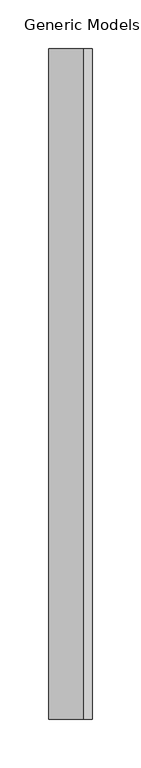
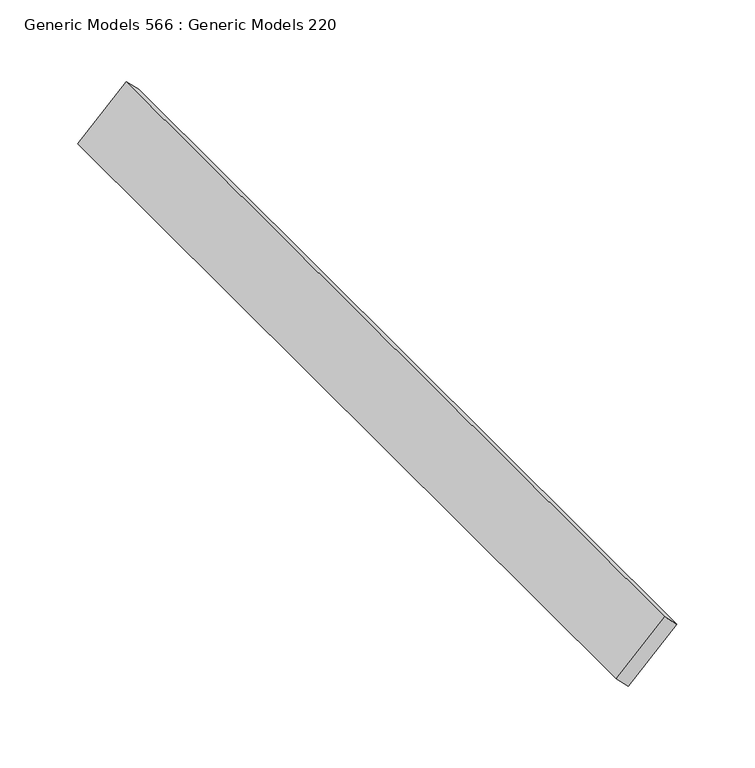
"""IFC4 building model written with IfcOpenShell, lengths in millimetres: proxy geometry, Generic Models 566 : Generic Models 220."""

from ifc_helpers import new_model, si_unit, frame, origin, place, context, project, spatial, polyline, outline, extrude, source, transform, mapped, element, save


def generic_models_566_generic_models_220_5707b333(model_context):
    return source(origin(), model_context, "Body", "SweptSolid", [
        extrude(outline(polyline([(0.0, -12.7000001), (0.0, 0.0), (690.8142348, 0.0), (690.8142348, -12.7000001), (0.0, -12.7000001)])), frame((7841.3059863, 4539.4872686, 124176.1399101), z_axis=(0.7071067811868034, 0.0, 0.7071067811862918), x_axis=(0.0, -1.0, 0.0)), (0.0, 0.0, 1.0), 50.8),
    ])


if __name__ == "__main__":
    model = new_model("IFC4")
    model_context = context("Model", 3, world=origin())
    ifc_project = project(units=[si_unit("LENGTHUNIT", "METRE", prefix="MILLI")], contexts=[model_context])
    site = spatial("IfcSite", under=ifc_project)
    building = spatial("IfcBuilding", under=site)
    placement = place(None, origin())
    generic_models_566_generic_models_220_shape = generic_models_566_generic_models_220_5707b333(model_context)
    element("IfcBuildingElementProxy", 1, Name="Generic Models 566 : Generic Models 220", ObjectType="Generic Models 566 : Generic Models 220", at=placement, inside=building, context=model_context, shape_type="MappedRepresentation", body=[
        mapped(generic_models_566_generic_models_220_shape, transform((0.0, 0.0, 0.0), x_axis=(1.0, 0.0, 0.0), y_axis=(0.0, 1.0, 0.0), z_axis=(0.0, 0.0, 1.0))),
    ])
    save(model, "model.ifc")

# Revit data of these elements
# Element 1 (IfcBuildingElementProxy, "Generic Models 566 : Generic Models 220")
#   Materials on its faces: "_WOOD TONE ALUMINUM EXTRUSION SLAT BY KNOTWOOD"
# Materials
#   "_WOOD TONE ALUMINUM EXTRUSION SLAT BY KNOTWOOD": class "Generic", colour RGB 177 130 114, transparency 0, Cost = 0
